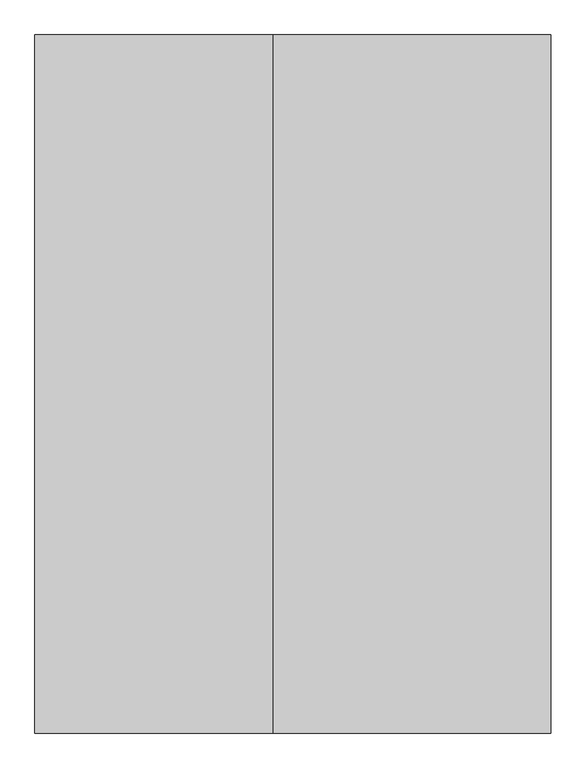
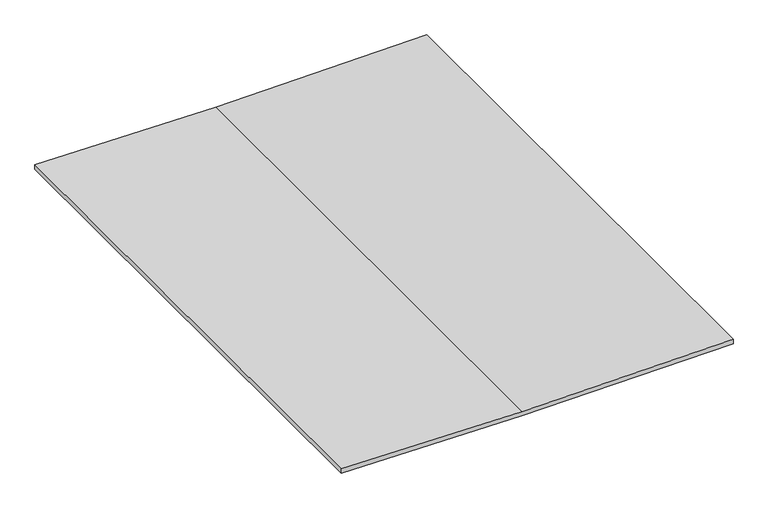
"""IFC4 building model written with IfcOpenShell, lengths in millimetres: proxy geometry, COVER BOARD2:COVER BOARD002:295712 : COVER BOARD2:COVER BOARD002:295712."""

from ifc_helpers import new_model, si_unit, frame, origin, place, context, project, spatial, polyline, outline, extrude, source, transform, mapped, element, save


def generic_models_54cbe6a4(model_context):
    return source(origin(), model_context, "Body", "SweptSolid", [
        extrude(outline(polyline([(40237.9000089, 3686.9275669), (40228.1021556, 2890.4461596), (40237.9000089, 2209.6354065), (40220.5682898, 2209.6354065), (40210.7704365, 2890.4461596), (40220.5682898, 3686.9275669), (40237.9000089, 3686.9275669)])), frame((0.0, 1278.3325411, 0.0), z_axis=(0.0, 1.0, 0.0), x_axis=(0.0, 0.0, 1.0)), (0.0, 0.0, 1.0), 2000.0),
    ])


if __name__ == "__main__":
    model = new_model("IFC4")
    model_context = context("Model", 3, world=origin())
    ifc_project = project(units=[si_unit("LENGTHUNIT", "METRE", prefix="MILLI")], contexts=[model_context])
    site = spatial("IfcSite", under=ifc_project)
    building = spatial("IfcBuilding", under=site)
    placement = place(None, origin())
    generic_models_shape = generic_models_54cbe6a4(model_context)
    element("IfcBuildingElementProxy", 1, Name="COVER BOARD2:COVER BOARD002:295712 : COVER BOARD2:COVER BOARD002:295712", ObjectType="COVER BOARD2:COVER BOARD002:295712 : COVER BOARD2:COVER BOARD002:295712", at=placement, inside=building, context=model_context, shape_type="MappedRepresentation", body=[
        mapped(generic_models_shape, transform((0.0, 0.0, 0.0), x_axis=(1.0, 0.0, 0.0), y_axis=(0.0, 1.0, 0.0), z_axis=(0.0, 0.0, 1.0))),
    ])
    save(model, "model.ifc")

# Revit data of these elements
# Type "COVER BOARD2:COVER BOARD002:295712 : COVER BOARD2:COVER BOARD002:295712"
#   NameOverride = "COVER BOARD2:COVER BOARD002:295712"
#   ObjectTypeOverride = "COVER BOARD2:COVER BOARD002"
#   Reference = "COVER BOARD002"
#   Category = "Generic Models"
#   Tag = "295712"
# Element 1 (IfcBuildingElementProxy, "COVER BOARD2:COVER BOARD002:295712 : COVER BOARD2:COVER BOARD002:295712")
#   Materials on its faces: "CDX PLYWOOD - SEE STRUCTURAL DWGS"
# Materials
#   "CDX PLYWOOD - SEE STRUCTURAL DWGS": class "Unassigned", colour RGB 202 163 108, transparency 0, Cost = 0
